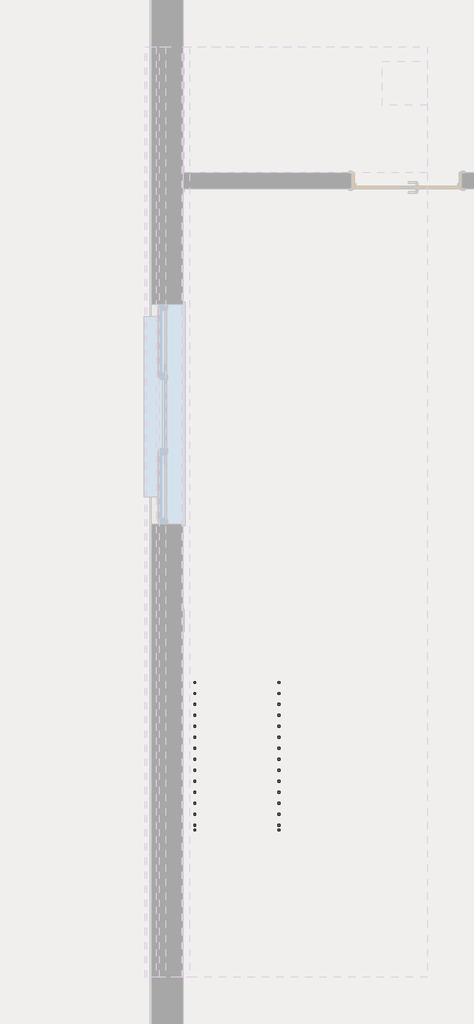
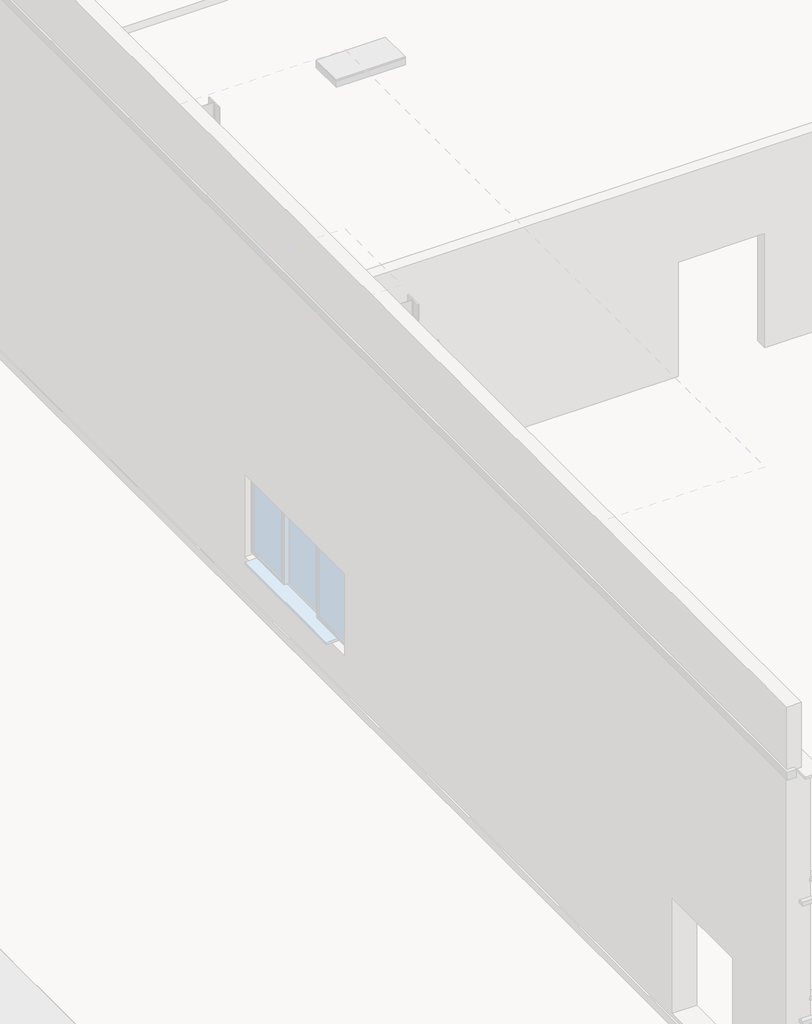
# One storey, part 7 of 13: 2 railings.
"""IFC4 building model written with IfcOpenShell, lengths in millimetres."""

from ifc_helpers import new_model, si_unit, frame, origin, place, context, project, spatial, polyline, outline, extrude, faceted_brep, element, save

model = new_model("IFC4")

# Units and contexts
model_context = context("Model", 3, world=origin())
ifc_project = project(units=[si_unit("LENGTHUNIT", "METRE", prefix="MILLI")], contexts=[model_context])

# Site, building, storey
site = spatial("IfcSite", under=ifc_project)
building = spatial("IfcBuilding", under=site)
storey = spatial("IfcBuildingStorey", under=building, Name="L0 - Ground Floor (Shadows On)", Elevation=0.0)

# Railings
placement = place(None, origin())
element("IfcRailing", 1, ObjectType="1100mm", at=placement, inside=storey, context=model_context, shape_type="SolidModel", body=[
    faceted_brep([(-5716.2916692, -13929.5546689, 1266.6666667), (-5716.2916692, -13929.5546689, 1209.4687214), (-5666.2916692, -13929.5546689, 1209.4687214), (-5666.2916692, -13929.5546689, 1266.6666667), (-5716.2916692, -11829.5546689, 2433.3333333), (-5716.2916692, -11816.5983675, 2383.3333333), (-5666.2916692, -11816.5983675, 2383.3333333), (-5666.2916692, -11829.5546689, 2433.3333333), (-5716.2916692, -10929.5546689, 2433.3333333), (-5716.2916692, -10916.5983675, 2383.3333333), (-5666.2916692, -10916.5983675, 2383.3333333), (-5666.2916692, -10929.5546689, 2433.3333333), (-5716.2916692, -8529.5546689, 3766.6666667), (-5716.2916692, -8516.5983675, 3716.6666667), (-5666.2916692, -8516.5983675, 3716.6666667), (-5666.2916692, -8529.5546689, 3766.6666667), (-5716.2916692, -7629.5546689, 3766.6666667), (-5716.2916692, -7616.5983675, 3716.6666667), (-5666.2916692, -7616.5983675, 3716.6666667), (-5666.2916692, -7629.5546689, 3766.6666667), (-5716.2916692, -5229.5546689, 5100.0), (-5666.2916692, -5229.5546689, 5100.0), (-5666.2916692, -5229.5546689, 5042.8020548), (-5716.2916692, -5229.5546689, 5042.8020548)], [[[0, 1, 2, 3]], [[1, 0, 4, 5]], [[2, 1, 5, 6]], [[3, 2, 6, 7]], [[0, 3, 7, 4]], [[5, 4, 8, 9]], [[6, 5, 9, 10]], [[7, 6, 10, 11]], [[4, 7, 11, 8]], [[9, 8, 12, 13]], [[10, 9, 13, 14]], [[11, 10, 14, 15]], [[8, 11, 15, 12]], [[13, 12, 16, 17]], [[14, 13, 17, 18]], [[15, 14, 18, 19]], [[12, 15, 19, 16]], [[20, 21, 22, 23]], [[17, 16, 20, 23]], [[18, 17, 23, 22]], [[19, 18, 22, 21]], [[16, 19, 21, 20]]]),
    extrude(outline(polyline([(-5317.0546689, 3833.3333333), (-5317.0546689, 4994.1909437), (-5292.0546689, 5008.0798326), (-5292.0546689, 3833.3333333), (-5317.0546689, 3833.3333333)])), frame((-5703.7916692, 0.0, 0.0), z_axis=(1.0, 0.0, 0.0), x_axis=(0.0, 1.0, 0.0)), (0.0, 0.0, 1.0), 25.0),
    extrude(outline(polyline([(-5467.0546689, 3833.3333333), (-5467.0546689, 4910.8576103), (-5442.0546689, 4924.7464992), (-5442.0546689, 3833.3333333), (-5467.0546689, 3833.3333333)])), frame((-5703.7916692, 0.0, 0.0), z_axis=(1.0, 0.0, 0.0), x_axis=(0.0, 1.0, 0.0)), (0.0, 0.0, 1.0), 25.0),
    extrude(outline(polyline([(-5617.0546689, 3666.6666667), (-5617.0546689, 4827.524277), (-5592.0546689, 4841.4131659), (-5592.0546689, 3666.6666667), (-5617.0546689, 3666.6666667)])), frame((-5703.7916692, 0.0, 0.0), z_axis=(1.0, 0.0, 0.0), x_axis=(0.0, 1.0, 0.0)), (0.0, 0.0, 1.0), 25.0),
    extrude(outline(polyline([(-5767.0546689, 3666.6666667), (-5767.0546689, 4744.1909437), (-5742.0546689, 4758.0798326), (-5742.0546689, 3666.6666667), (-5767.0546689, 3666.6666667)])), frame((-5703.7916692, 0.0, 0.0), z_axis=(1.0, 0.0, 0.0), x_axis=(0.0, 1.0, 0.0)), (0.0, 0.0, 1.0), 25.0),
    extrude(outline(polyline([(-5917.0546689, 3500.0), (-5917.0546689, 4660.8576103), (-5892.0546689, 4674.7464992), (-5892.0546689, 3500.0), (-5917.0546689, 3500.0)])), frame((-5703.7916692, 0.0, 0.0), z_axis=(1.0, 0.0, 0.0), x_axis=(0.0, 1.0, 0.0)), (0.0, 0.0, 1.0), 25.0),
    extrude(outline(polyline([(-6067.0546689, 3500.0), (-6067.0546689, 4577.524277), (-6042.0546689, 4591.4131659), (-6042.0546689, 3500.0), (-6067.0546689, 3500.0)])), frame((-5703.7916692, 0.0, 0.0), z_axis=(1.0, 0.0, 0.0), x_axis=(0.0, 1.0, 0.0)), (0.0, 0.0, 1.0), 25.0),
    extrude(outline(polyline([(-6217.0546689, 3333.3333333), (-6217.0546689, 4494.1909437), (-6192.0546689, 4508.0798326), (-6192.0546689, 3333.3333333), (-6217.0546689, 3333.3333333)])), frame((-5703.7916692, 0.0, 0.0), z_axis=(1.0, 0.0, 0.0), x_axis=(0.0, 1.0, 0.0)), (0.0, 0.0, 1.0), 25.0),
    extrude(outline(polyline([(-6367.0546689, 3333.3333333), (-6367.0546689, 4410.8576103), (-6342.0546689, 4424.7464992), (-6342.0546689, 3333.3333333), (-6367.0546689, 3333.3333333)])), frame((-5703.7916692, 0.0, 0.0), z_axis=(1.0, 0.0, 0.0), x_axis=(0.0, 1.0, 0.0)), (0.0, 0.0, 1.0), 25.0),
    extrude(outline(polyline([(-6517.0546689, 3166.6666667), (-6517.0546689, 4327.524277), (-6492.0546689, 4341.4131659), (-6492.0546689, 3166.6666667), (-6517.0546689, 3166.6666667)])), frame((-5703.7916692, 0.0, 0.0), z_axis=(1.0, 0.0, 0.0), x_axis=(0.0, 1.0, 0.0)), (0.0, 0.0, 1.0), 25.0),
    extrude(outline(polyline([(-6667.0546689, 3166.6666667), (-6667.0546689, 4244.1909437), (-6642.0546689, 4258.0798326), (-6642.0546689, 3166.6666667), (-6667.0546689, 3166.6666667)])), frame((-5703.7916692, 0.0, 0.0), z_axis=(1.0, 0.0, 0.0), x_axis=(0.0, 1.0, 0.0)), (0.0, 0.0, 1.0), 25.0),
    extrude(outline(polyline([(-6817.0546689, 3000.0), (-6817.0546689, 4160.8576103), (-6792.0546689, 4174.7464992), (-6792.0546689, 3000.0), (-6817.0546689, 3000.0)])), frame((-5703.7916692, 0.0, 0.0), z_axis=(1.0, 0.0, 0.0), x_axis=(0.0, 1.0, 0.0)), (0.0, 0.0, 1.0), 25.0),
    extrude(outline(polyline([(-6967.0546689, 3000.0), (-6967.0546689, 4077.524277), (-6942.0546689, 4091.4131659), (-6942.0546689, 3000.0), (-6967.0546689, 3000.0)])), frame((-5703.7916692, 0.0, 0.0), z_axis=(1.0, 0.0, 0.0), x_axis=(0.0, 1.0, 0.0)), (0.0, 0.0, 1.0), 25.0),
    extrude(outline(polyline([(-7117.0546689, 2833.3333333), (-7117.0546689, 3994.1909437), (-7092.0546689, 4008.0798326), (-7092.0546689, 2833.3333333), (-7117.0546689, 2833.3333333)])), frame((-5703.7916692, 0.0, 0.0), z_axis=(1.0, 0.0, 0.0), x_axis=(0.0, 1.0, 0.0)), (0.0, 0.0, 1.0), 25.0),
    extrude(outline(polyline([(-7267.0546689, 2833.3333333), (-7267.0546689, 3910.8576103), (-7242.0546689, 3924.7464992), (-7242.0546689, 2833.3333333), (-7267.0546689, 2833.3333333)])), frame((-5703.7916692, 0.0, 0.0), z_axis=(1.0, 0.0, 0.0), x_axis=(0.0, 1.0, 0.0)), (0.0, 0.0, 1.0), 25.0),
    extrude(outline(polyline([(-7417.0546689, 2666.6666667), (-7417.0546689, 3827.524277), (-7392.0546689, 3841.4131659), (-7392.0546689, 2666.6666667), (-7417.0546689, 2666.6666667)])), frame((-5703.7916692, 0.0, 0.0), z_axis=(1.0, 0.0, 0.0), x_axis=(0.0, 1.0, 0.0)), (0.0, 0.0, 1.0), 25.0),
    extrude(outline(polyline([(-7567.0546689, 2666.6666667), (-7567.0546689, 3744.1909437), (-7542.0546689, 3758.0798326), (-7542.0546689, 2666.6666667), (-7567.0546689, 2666.6666667)])), frame((-5703.7916692, 0.0, 0.0), z_axis=(1.0, 0.0, 0.0), x_axis=(0.0, 1.0, 0.0)), (0.0, 0.0, 1.0), 25.0),
    extrude(outline(polyline([(-5678.7916692, -7717.0546689), (-5703.7916692, -7717.0546689), (-5703.7916692, -7692.0546689), (-5678.7916692, -7692.0546689), (-5678.7916692, -7717.0546689)])), frame((0.0, 0.0, 2666.6666667), z_axis=(0.0, 0.0, 1.0), x_axis=(1.0, 0.0, 0.0)), (0.0, 0.0, 1.0), 1050.0),
    extrude(outline(polyline([(-5678.7916692, -7867.0546689), (-5703.7916692, -7867.0546689), (-5703.7916692, -7842.0546689), (-5678.7916692, -7842.0546689), (-5678.7916692, -7867.0546689)])), frame((0.0, 0.0, 2666.6666667), z_axis=(0.0, 0.0, 1.0), x_axis=(1.0, 0.0, 0.0)), (0.0, 0.0, 1.0), 1050.0),
    extrude(outline(polyline([(-5678.7916692, -8017.0546689), (-5703.7916692, -8017.0546689), (-5703.7916692, -7992.0546689), (-5678.7916692, -7992.0546689), (-5678.7916692, -8017.0546689)])), frame((0.0, 0.0, 2666.6666667), z_axis=(0.0, 0.0, 1.0), x_axis=(1.0, 0.0, 0.0)), (0.0, 0.0, 1.0), 1050.0),
    extrude(outline(polyline([(-5678.7916692, -8167.0546689), (-5703.7916692, -8167.0546689), (-5703.7916692, -8142.0546689), (-5678.7916692, -8142.0546689), (-5678.7916692, -8167.0546689)])), frame((0.0, 0.0, 2666.6666667), z_axis=(0.0, 0.0, 1.0), x_axis=(1.0, 0.0, 0.0)), (0.0, 0.0, 1.0), 1050.0),
    extrude(outline(polyline([(-5678.7916692, -8317.0546689), (-5703.7916692, -8317.0546689), (-5703.7916692, -8292.0546689), (-5678.7916692, -8292.0546689), (-5678.7916692, -8317.0546689)])), frame((0.0, 0.0, 2666.6666667), z_axis=(0.0, 0.0, 1.0), x_axis=(1.0, 0.0, 0.0)), (0.0, 0.0, 1.0), 1050.0),
    extrude(outline(polyline([(-5678.7916692, -8467.0546689), (-5703.7916692, -8467.0546689), (-5703.7916692, -8442.0546689), (-5678.7916692, -8442.0546689), (-5678.7916692, -8467.0546689)])), frame((0.0, 0.0, 2666.6666667), z_axis=(0.0, 0.0, 1.0), x_axis=(1.0, 0.0, 0.0)), (0.0, 0.0, 1.0), 1050.0),
    extrude(outline(polyline([(-8617.0546689, 2500.0), (-8617.0546689, 3660.8576103), (-8592.0546689, 3674.7464992), (-8592.0546689, 2500.0), (-8617.0546689, 2500.0)])), frame((-5703.7916692, 0.0, 0.0), z_axis=(1.0, 0.0, 0.0), x_axis=(0.0, 1.0, 0.0)), (0.0, 0.0, 1.0), 25.0),
    extrude(outline(polyline([(-8767.0546689, 2500.0), (-8767.0546689, 3577.524277), (-8742.0546689, 3591.4131659), (-8742.0546689, 2500.0), (-8767.0546689, 2500.0)])), frame((-5703.7916692, 0.0, 0.0), z_axis=(1.0, 0.0, 0.0), x_axis=(0.0, 1.0, 0.0)), (0.0, 0.0, 1.0), 25.0),
    extrude(outline(polyline([(-8917.0546689, 2333.3333333), (-8917.0546689, 3494.1909437), (-8892.0546689, 3508.0798326), (-8892.0546689, 2333.3333333), (-8917.0546689, 2333.3333333)])), frame((-5703.7916692, 0.0, 0.0), z_axis=(1.0, 0.0, 0.0), x_axis=(0.0, 1.0, 0.0)), (0.0, 0.0, 1.0), 25.0),
    extrude(outline(polyline([(-9067.0546689, 2333.3333333), (-9067.0546689, 3410.8576103), (-9042.0546689, 3424.7464992), (-9042.0546689, 2333.3333333), (-9067.0546689, 2333.3333333)])), frame((-5703.7916692, 0.0, 0.0), z_axis=(1.0, 0.0, 0.0), x_axis=(0.0, 1.0, 0.0)), (0.0, 0.0, 1.0), 25.0),
    extrude(outline(polyline([(-9217.0546689, 2166.6666667), (-9217.0546689, 3327.524277), (-9192.0546689, 3341.4131659), (-9192.0546689, 2166.6666667), (-9217.0546689, 2166.6666667)])), frame((-5703.7916692, 0.0, 0.0), z_axis=(1.0, 0.0, 0.0), x_axis=(0.0, 1.0, 0.0)), (0.0, 0.0, 1.0), 25.0),
    extrude(outline(polyline([(-9367.0546689, 2166.6666667), (-9367.0546689, 3244.1909437), (-9342.0546689, 3258.0798326), (-9342.0546689, 2166.6666667), (-9367.0546689, 2166.6666667)])), frame((-5703.7916692, 0.0, 0.0), z_axis=(1.0, 0.0, 0.0), x_axis=(0.0, 1.0, 0.0)), (0.0, 0.0, 1.0), 25.0),
    extrude(outline(polyline([(-9517.0546689, 2000.0), (-9517.0546689, 3160.8576103), (-9492.0546689, 3174.7464992), (-9492.0546689, 2000.0), (-9517.0546689, 2000.0)])), frame((-5703.7916692, 0.0, 0.0), z_axis=(1.0, 0.0, 0.0), x_axis=(0.0, 1.0, 0.0)), (0.0, 0.0, 1.0), 25.0),
    extrude(outline(polyline([(-9667.0546689, 2000.0), (-9667.0546689, 3077.524277), (-9642.0546689, 3091.4131659), (-9642.0546689, 2000.0), (-9667.0546689, 2000.0)])), frame((-5703.7916692, 0.0, 0.0), z_axis=(1.0, 0.0, 0.0), x_axis=(0.0, 1.0, 0.0)), (0.0, 0.0, 1.0), 25.0),
    extrude(outline(polyline([(-9817.0546689, 1833.3333333), (-9817.0546689, 2994.1909437), (-9792.0546689, 3008.0798326), (-9792.0546689, 1833.3333333), (-9817.0546689, 1833.3333333)])), frame((-5703.7916692, 0.0, 0.0), z_axis=(1.0, 0.0, 0.0), x_axis=(0.0, 1.0, 0.0)), (0.0, 0.0, 1.0), 25.0),
    extrude(outline(polyline([(-9967.0546689, 1833.3333333), (-9967.0546689, 2910.8576103), (-9942.0546689, 2924.7464992), (-9942.0546689, 1833.3333333), (-9967.0546689, 1833.3333333)])), frame((-5703.7916692, 0.0, 0.0), z_axis=(1.0, 0.0, 0.0), x_axis=(0.0, 1.0, 0.0)), (0.0, 0.0, 1.0), 25.0),
    extrude(outline(polyline([(-10117.0546689, 1666.6666667), (-10117.0546689, 2827.524277), (-10092.0546689, 2841.4131659), (-10092.0546689, 1666.6666667), (-10117.0546689, 1666.6666667)])), frame((-5703.7916692, 0.0, 0.0), z_axis=(1.0, 0.0, 0.0), x_axis=(0.0, 1.0, 0.0)), (0.0, 0.0, 1.0), 25.0),
    extrude(outline(polyline([(-10267.0546689, 1666.6666667), (-10267.0546689, 2744.1909437), (-10242.0546689, 2758.0798326), (-10242.0546689, 1666.6666667), (-10267.0546689, 1666.6666667)])), frame((-5703.7916692, 0.0, 0.0), z_axis=(1.0, 0.0, 0.0), x_axis=(0.0, 1.0, 0.0)), (0.0, 0.0, 1.0), 25.0),
    extrude(outline(polyline([(-10417.0546689, 1500.0), (-10417.0546689, 2660.8576103), (-10392.0546689, 2674.7464992), (-10392.0546689, 1500.0), (-10417.0546689, 1500.0)])), frame((-5703.7916692, 0.0, 0.0), z_axis=(1.0, 0.0, 0.0), x_axis=(0.0, 1.0, 0.0)), (0.0, 0.0, 1.0), 25.0),
    extrude(outline(polyline([(-10567.0546689, 1500.0), (-10567.0546689, 2577.524277), (-10542.0546689, 2591.4131659), (-10542.0546689, 1500.0), (-10567.0546689, 1500.0)])), frame((-5703.7916692, 0.0, 0.0), z_axis=(1.0, 0.0, 0.0), x_axis=(0.0, 1.0, 0.0)), (0.0, 0.0, 1.0), 25.0),
    extrude(outline(polyline([(-10717.0546689, 1333.3333333), (-10717.0546689, 2494.1909437), (-10692.0546689, 2508.0798326), (-10692.0546689, 1333.3333333), (-10717.0546689, 1333.3333333)])), frame((-5703.7916692, 0.0, 0.0), z_axis=(1.0, 0.0, 0.0), x_axis=(0.0, 1.0, 0.0)), (0.0, 0.0, 1.0), 25.0),
    extrude(outline(polyline([(-10867.0546689, 1333.3333333), (-10867.0546689, 2410.8576103), (-10842.0546689, 2424.7464992), (-10842.0546689, 1333.3333333), (-10867.0546689, 1333.3333333)])), frame((-5703.7916692, 0.0, 0.0), z_axis=(1.0, 0.0, 0.0), x_axis=(0.0, 1.0, 0.0)), (0.0, 0.0, 1.0), 25.0),
    extrude(outline(polyline([(-5678.7916692, -11017.0546689), (-5703.7916692, -11017.0546689), (-5703.7916692, -10992.0546689), (-5678.7916692, -10992.0546689), (-5678.7916692, -11017.0546689)])), frame((0.0, 0.0, 1333.3333333), z_axis=(0.0, 0.0, 1.0), x_axis=(1.0, 0.0, 0.0)), (0.0, 0.0, 1.0), 1050.0),
    extrude(outline(polyline([(-5678.7916692, -11167.0546689), (-5703.7916692, -11167.0546689), (-5703.7916692, -11142.0546689), (-5678.7916692, -11142.0546689), (-5678.7916692, -11167.0546689)])), frame((0.0, 0.0, 1333.3333333), z_axis=(0.0, 0.0, 1.0), x_axis=(1.0, 0.0, 0.0)), (0.0, 0.0, 1.0), 1050.0),
    extrude(outline(polyline([(-5678.7916692, -11317.0546689), (-5703.7916692, -11317.0546689), (-5703.7916692, -11292.0546689), (-5678.7916692, -11292.0546689), (-5678.7916692, -11317.0546689)])), frame((0.0, 0.0, 1333.3333333), z_axis=(0.0, 0.0, 1.0), x_axis=(1.0, 0.0, 0.0)), (0.0, 0.0, 1.0), 1050.0),
    extrude(outline(polyline([(-5678.7916692, -11467.0546689), (-5703.7916692, -11467.0546689), (-5703.7916692, -11442.0546689), (-5678.7916692, -11442.0546689), (-5678.7916692, -11467.0546689)])), frame((0.0, 0.0, 1333.3333333), z_axis=(0.0, 0.0, 1.0), x_axis=(1.0, 0.0, 0.0)), (0.0, 0.0, 1.0), 1050.0),
    extrude(outline(polyline([(-5678.7916692, -11617.0546689), (-5703.7916692, -11617.0546689), (-5703.7916692, -11592.0546689), (-5678.7916692, -11592.0546689), (-5678.7916692, -11617.0546689)])), frame((0.0, 0.0, 1333.3333333), z_axis=(0.0, 0.0, 1.0), x_axis=(1.0, 0.0, 0.0)), (0.0, 0.0, 1.0), 1050.0),
    extrude(outline(polyline([(-5678.7916692, -11767.0546689), (-5703.7916692, -11767.0546689), (-5703.7916692, -11742.0546689), (-5678.7916692, -11742.0546689), (-5678.7916692, -11767.0546689)])), frame((0.0, 0.0, 1333.3333333), z_axis=(0.0, 0.0, 1.0), x_axis=(1.0, 0.0, 0.0)), (0.0, 0.0, 1.0), 1050.0),
    extrude(outline(polyline([(-11917.0546689, 1166.6666667), (-11917.0546689, 2327.524277), (-11892.0546689, 2341.4131659), (-11892.0546689, 1166.6666667), (-11917.0546689, 1166.6666667)])), frame((-5703.7916692, 0.0, 0.0), z_axis=(1.0, 0.0, 0.0), x_axis=(0.0, 1.0, 0.0)), (0.0, 0.0, 1.0), 25.0),
    extrude(outline(polyline([(-12067.0546689, 1166.6666667), (-12067.0546689, 2244.1909437), (-12042.0546689, 2258.0798326), (-12042.0546689, 1166.6666667), (-12067.0546689, 1166.6666667)])), frame((-5703.7916692, 0.0, 0.0), z_axis=(1.0, 0.0, 0.0), x_axis=(0.0, 1.0, 0.0)), (0.0, 0.0, 1.0), 25.0),
    extrude(outline(polyline([(-12217.0546689, 1000.0), (-12217.0546689, 2160.8576103), (-12192.0546689, 2174.7464992), (-12192.0546689, 1000.0), (-12217.0546689, 1000.0)])), frame((-5703.7916692, 0.0, 0.0), z_axis=(1.0, 0.0, 0.0), x_axis=(0.0, 1.0, 0.0)), (0.0, 0.0, 1.0), 25.0),
    extrude(outline(polyline([(-12367.0546689, 1000.0), (-12367.0546689, 2077.524277), (-12342.0546689, 2091.4131659), (-12342.0546689, 1000.0), (-12367.0546689, 1000.0)])), frame((-5703.7916692, 0.0, 0.0), z_axis=(1.0, 0.0, 0.0), x_axis=(0.0, 1.0, 0.0)), (0.0, 0.0, 1.0), 25.0),
    extrude(outline(polyline([(-12517.0546689, 833.3333333), (-12517.0546689, 1994.1909437), (-12492.0546689, 2008.0798326), (-12492.0546689, 833.3333333), (-12517.0546689, 833.3333333)])), frame((-5703.7916692, 0.0, 0.0), z_axis=(1.0, 0.0, 0.0), x_axis=(0.0, 1.0, 0.0)), (0.0, 0.0, 1.0), 25.0),
    extrude(outline(polyline([(-12667.0546689, 833.3333333), (-12667.0546689, 1910.8576103), (-12642.0546689, 1924.7464992), (-12642.0546689, 833.3333333), (-12667.0546689, 833.3333333)])), frame((-5703.7916692, 0.0, 0.0), z_axis=(1.0, 0.0, 0.0), x_axis=(0.0, 1.0, 0.0)), (0.0, 0.0, 1.0), 25.0),
    extrude(outline(polyline([(-12817.0546689, 666.6666667), (-12817.0546689, 1827.524277), (-12792.0546689, 1841.4131659), (-12792.0546689, 666.6666667), (-12817.0546689, 666.6666667)])), frame((-5703.7916692, 0.0, 0.0), z_axis=(1.0, 0.0, 0.0), x_axis=(0.0, 1.0, 0.0)), (0.0, 0.0, 1.0), 25.0),
    extrude(outline(polyline([(-12967.0546689, 666.6666667), (-12967.0546689, 1744.1909437), (-12942.0546689, 1758.0798326), (-12942.0546689, 666.6666667), (-12967.0546689, 666.6666667)])), frame((-5703.7916692, 0.0, 0.0), z_axis=(1.0, 0.0, 0.0), x_axis=(0.0, 1.0, 0.0)), (0.0, 0.0, 1.0), 25.0),
    extrude(outline(polyline([(-13117.0546689, 500.0), (-13117.0546689, 1660.8576103), (-13092.0546689, 1674.7464992), (-13092.0546689, 500.0), (-13117.0546689, 500.0)])), frame((-5703.7916692, 0.0, 0.0), z_axis=(1.0, 0.0, 0.0), x_axis=(0.0, 1.0, 0.0)), (0.0, 0.0, 1.0), 25.0),
    extrude(outline(polyline([(-13267.0546689, 500.0), (-13267.0546689, 1577.524277), (-13242.0546689, 1591.4131659), (-13242.0546689, 500.0), (-13267.0546689, 500.0)])), frame((-5703.7916692, 0.0, 0.0), z_axis=(1.0, 0.0, 0.0), x_axis=(0.0, 1.0, 0.0)), (0.0, 0.0, 1.0), 25.0),
    extrude(outline(polyline([(-13417.0546689, 333.3333333), (-13417.0546689, 1494.1909437), (-13392.0546689, 1508.0798326), (-13392.0546689, 333.3333333), (-13417.0546689, 333.3333333)])), frame((-5703.7916692, 0.0, 0.0), z_axis=(1.0, 0.0, 0.0), x_axis=(0.0, 1.0, 0.0)), (0.0, 0.0, 1.0), 25.0),
    extrude(outline(polyline([(-13567.0546689, 333.3333333), (-13567.0546689, 1410.8576103), (-13542.0546689, 1424.7464992), (-13542.0546689, 333.3333333), (-13567.0546689, 333.3333333)])), frame((-5703.7916692, 0.0, 0.0), z_axis=(1.0, 0.0, 0.0), x_axis=(0.0, 1.0, 0.0)), (0.0, 0.0, 1.0), 25.0),
    extrude(outline(polyline([(-13717.0546689, 166.6666667), (-13717.0546689, 1327.524277), (-13692.0546689, 1341.4131659), (-13692.0546689, 166.6666667), (-13717.0546689, 166.6666667)])), frame((-5703.7916692, 0.0, 0.0), z_axis=(1.0, 0.0, 0.0), x_axis=(0.0, 1.0, 0.0)), (0.0, 0.0, 1.0), 25.0),
    extrude(outline(polyline([(-13867.0546689, 166.6666667), (-13867.0546689, 1244.1909437), (-13842.0546689, 1258.0798326), (-13842.0546689, 166.6666667), (-13867.0546689, 166.6666667)])), frame((-5703.7916692, 0.0, 0.0), z_axis=(1.0, 0.0, 0.0), x_axis=(0.0, 1.0, 0.0)), (0.0, 0.0, 1.0), 25.0),
    extrude(outline(polyline([(-5678.7916692, -7642.0546689), (-5703.7916692, -7642.0546689), (-5703.7916692, -7617.0546689), (-5678.7916692, -7617.0546689), (-5678.7916692, -7642.0546689)])), frame((0.0, 0.0, 2666.6666667), z_axis=(0.0, 0.0, 1.0), x_axis=(1.0, 0.0, 0.0)), (0.0, 0.0, 1.0), 1050.0),
    extrude(outline(polyline([(-8542.0546689, 2666.6666667), (-8542.0546689, 3702.524277), (-8517.0546689, 3716.4131659), (-8517.0546689, 2666.6666667), (-8542.0546689, 2666.6666667)])), frame((-5703.7916692, 0.0, 0.0), z_axis=(1.0, 0.0, 0.0), x_axis=(0.0, 1.0, 0.0)), (0.0, 0.0, 1.0), 25.0),
    extrude(outline(polyline([(-5678.7916692, -10942.0546689), (-5703.7916692, -10942.0546689), (-5703.7916692, -10917.0546689), (-5678.7916692, -10917.0546689), (-5678.7916692, -10942.0546689)])), frame((0.0, 0.0, 1333.3333333), z_axis=(0.0, 0.0, 1.0), x_axis=(1.0, 0.0, 0.0)), (0.0, 0.0, 1.0), 1050.0),
    extrude(outline(polyline([(-11842.0546689, 1333.3333333), (-11842.0546689, 2369.1909437), (-11817.0546689, 2383.0798326), (-11817.0546689, 1333.3333333), (-11842.0546689, 1333.3333333)])), frame((-5703.7916692, 0.0, 0.0), z_axis=(1.0, 0.0, 0.0), x_axis=(0.0, 1.0, 0.0)), (0.0, 0.0, 1.0), 25.0),
    extrude(outline(polyline([(-5254.5546689, 3833.3333333), (-5254.5546689, 5028.9131659), (-5229.5546689, 5042.8020548), (-5229.5546689, 3833.3333333), (-5254.5546689, 3833.3333333)])), frame((-5703.7916692, 0.0, 0.0), z_axis=(1.0, 0.0, 0.0), x_axis=(0.0, 1.0, 0.0)), (0.0, 0.0, 1.0), 25.0),
    extrude(outline(polyline([(-13929.5546689, 166.6666667), (-13929.5546689, 1209.4687214), (-13904.5546689, 1223.3576103), (-13904.5546689, 166.6666667), (-13929.5546689, 166.6666667)])), frame((-5703.7916692, 0.0, 0.0), z_axis=(1.0, 0.0, 0.0), x_axis=(0.0, 1.0, 0.0)), (0.0, 0.0, 1.0), 25.0),
])
element("IfcRailing", 2, ObjectType="1100mm", at=placement, inside=storey, context=model_context, shape_type="SolidModel", body=[
    faceted_brep([(-6865.4916692, -13929.5546689, 1266.6666667), (-6865.4916692, -13929.5546689, 1209.4687214), (-6815.4916692, -13929.5546689, 1209.4687214), (-6815.4916692, -13929.5546689, 1266.6666667), (-6865.4916692, -11829.5546689, 2433.3333333), (-6865.4916692, -11816.5983675, 2383.3333333), (-6815.4916692, -11816.5983675, 2383.3333333), (-6815.4916692, -11829.5546689, 2433.3333333), (-6865.4916692, -10929.5546689, 2433.3333333), (-6865.4916692, -10916.5983675, 2383.3333333), (-6815.4916692, -10916.5983675, 2383.3333333), (-6815.4916692, -10929.5546689, 2433.3333333), (-6865.4916692, -8529.5546689, 3766.6666667), (-6865.4916692, -8516.5983675, 3716.6666667), (-6815.4916692, -8516.5983675, 3716.6666667), (-6815.4916692, -8529.5546689, 3766.6666667), (-6865.4916692, -7629.5546689, 3766.6666667), (-6865.4916692, -7616.5983675, 3716.6666667), (-6815.4916692, -7616.5983675, 3716.6666667), (-6815.4916692, -7629.5546689, 3766.6666667), (-6865.4916692, -5229.5546689, 5100.0), (-6815.4916692, -5229.5546689, 5100.0), (-6815.4916692, -5229.5546689, 5042.8020548), (-6865.4916692, -5229.5546689, 5042.8020548)], [[[0, 1, 2, 3]], [[1, 0, 4, 5]], [[2, 1, 5, 6]], [[3, 2, 6, 7]], [[0, 3, 7, 4]], [[5, 4, 8, 9]], [[6, 5, 9, 10]], [[7, 6, 10, 11]], [[4, 7, 11, 8]], [[9, 8, 12, 13]], [[10, 9, 13, 14]], [[11, 10, 14, 15]], [[8, 11, 15, 12]], [[13, 12, 16, 17]], [[14, 13, 17, 18]], [[15, 14, 18, 19]], [[12, 15, 19, 16]], [[20, 21, 22, 23]], [[17, 16, 20, 23]], [[18, 17, 23, 22]], [[19, 18, 22, 21]], [[16, 19, 21, 20]]]),
    extrude(outline(polyline([(-5317.0546689, 4994.1909437), (-5292.0546689, 5008.0798326), (-5292.0546689, 3833.3333333), (-5317.0546689, 3833.3333333), (-5317.0546689, 4994.1909437)])), frame((-6852.9916692, 0.0, 0.0), z_axis=(1.0, 0.0, 0.0), x_axis=(0.0, 1.0, 0.0)), (0.0, 0.0, 1.0), 25.0),
    extrude(outline(polyline([(-5467.0546689, 4910.8576103), (-5442.0546689, 4924.7464992), (-5442.0546689, 3833.3333333), (-5467.0546689, 3833.3333333), (-5467.0546689, 4910.8576103)])), frame((-6852.9916692, 0.0, 0.0), z_axis=(1.0, 0.0, 0.0), x_axis=(0.0, 1.0, 0.0)), (0.0, 0.0, 1.0), 25.0),
    extrude(outline(polyline([(-5617.0546689, 4827.524277), (-5592.0546689, 4841.4131659), (-5592.0546689, 3666.6666667), (-5617.0546689, 3666.6666667), (-5617.0546689, 4827.524277)])), frame((-6852.9916692, 0.0, 0.0), z_axis=(1.0, 0.0, 0.0), x_axis=(0.0, 1.0, 0.0)), (0.0, 0.0, 1.0), 25.0),
    extrude(outline(polyline([(-5767.0546689, 4744.1909437), (-5742.0546689, 4758.0798326), (-5742.0546689, 3666.6666667), (-5767.0546689, 3666.6666667), (-5767.0546689, 4744.1909437)])), frame((-6852.9916692, 0.0, 0.0), z_axis=(1.0, 0.0, 0.0), x_axis=(0.0, 1.0, 0.0)), (0.0, 0.0, 1.0), 25.0),
    extrude(outline(polyline([(-5917.0546689, 4660.8576103), (-5892.0546689, 4674.7464992), (-5892.0546689, 3500.0), (-5917.0546689, 3500.0), (-5917.0546689, 4660.8576103)])), frame((-6852.9916692, 0.0, 0.0), z_axis=(1.0, 0.0, 0.0), x_axis=(0.0, 1.0, 0.0)), (0.0, 0.0, 1.0), 25.0),
    extrude(outline(polyline([(-6067.0546689, 4577.524277), (-6042.0546689, 4591.4131659), (-6042.0546689, 3500.0), (-6067.0546689, 3500.0), (-6067.0546689, 4577.524277)])), frame((-6852.9916692, 0.0, 0.0), z_axis=(1.0, 0.0, 0.0), x_axis=(0.0, 1.0, 0.0)), (0.0, 0.0, 1.0), 25.0),
    extrude(outline(polyline([(-6217.0546689, 4494.1909437), (-6192.0546689, 4508.0798326), (-6192.0546689, 3333.3333333), (-6217.0546689, 3333.3333333), (-6217.0546689, 4494.1909437)])), frame((-6852.9916692, 0.0, 0.0), z_axis=(1.0, 0.0, 0.0), x_axis=(0.0, 1.0, 0.0)), (0.0, 0.0, 1.0), 25.0),
    extrude(outline(polyline([(-6367.0546689, 4410.8576103), (-6342.0546689, 4424.7464992), (-6342.0546689, 3333.3333333), (-6367.0546689, 3333.3333333), (-6367.0546689, 4410.8576103)])), frame((-6852.9916692, 0.0, 0.0), z_axis=(1.0, 0.0, 0.0), x_axis=(0.0, 1.0, 0.0)), (0.0, 0.0, 1.0), 25.0),
    extrude(outline(polyline([(-6517.0546689, 4327.524277), (-6492.0546689, 4341.4131659), (-6492.0546689, 3166.6666667), (-6517.0546689, 3166.6666667), (-6517.0546689, 4327.524277)])), frame((-6852.9916692, 0.0, 0.0), z_axis=(1.0, 0.0, 0.0), x_axis=(0.0, 1.0, 0.0)), (0.0, 0.0, 1.0), 25.0),
    extrude(outline(polyline([(-6667.0546689, 4244.1909437), (-6642.0546689, 4258.0798326), (-6642.0546689, 3166.6666667), (-6667.0546689, 3166.6666667), (-6667.0546689, 4244.1909437)])), frame((-6852.9916692, 0.0, 0.0), z_axis=(1.0, 0.0, 0.0), x_axis=(0.0, 1.0, 0.0)), (0.0, 0.0, 1.0), 25.0),
    extrude(outline(polyline([(-6817.0546689, 4160.8576103), (-6792.0546689, 4174.7464992), (-6792.0546689, 3000.0), (-6817.0546689, 3000.0), (-6817.0546689, 4160.8576103)])), frame((-6852.9916692, 0.0, 0.0), z_axis=(1.0, 0.0, 0.0), x_axis=(0.0, 1.0, 0.0)), (0.0, 0.0, 1.0), 25.0),
    extrude(outline(polyline([(-6967.0546689, 4077.524277), (-6942.0546689, 4091.4131659), (-6942.0546689, 3000.0), (-6967.0546689, 3000.0), (-6967.0546689, 4077.524277)])), frame((-6852.9916692, 0.0, 0.0), z_axis=(1.0, 0.0, 0.0), x_axis=(0.0, 1.0, 0.0)), (0.0, 0.0, 1.0), 25.0),
    extrude(outline(polyline([(-7117.0546689, 3994.1909437), (-7092.0546689, 4008.0798326), (-7092.0546689, 2833.3333333), (-7117.0546689, 2833.3333333), (-7117.0546689, 3994.1909437)])), frame((-6852.9916692, 0.0, 0.0), z_axis=(1.0, 0.0, 0.0), x_axis=(0.0, 1.0, 0.0)), (0.0, 0.0, 1.0), 25.0),
    extrude(outline(polyline([(-7267.0546689, 3910.8576103), (-7242.0546689, 3924.7464992), (-7242.0546689, 2833.3333333), (-7267.0546689, 2833.3333333), (-7267.0546689, 3910.8576103)])), frame((-6852.9916692, 0.0, 0.0), z_axis=(1.0, 0.0, 0.0), x_axis=(0.0, 1.0, 0.0)), (0.0, 0.0, 1.0), 25.0),
    extrude(outline(polyline([(-7417.0546689, 3827.524277), (-7392.0546689, 3841.4131659), (-7392.0546689, 2666.6666667), (-7417.0546689, 2666.6666667), (-7417.0546689, 3827.524277)])), frame((-6852.9916692, 0.0, 0.0), z_axis=(1.0, 0.0, 0.0), x_axis=(0.0, 1.0, 0.0)), (0.0, 0.0, 1.0), 25.0),
    extrude(outline(polyline([(-7567.0546689, 3744.1909437), (-7542.0546689, 3758.0798326), (-7542.0546689, 2666.6666667), (-7567.0546689, 2666.6666667), (-7567.0546689, 3744.1909437)])), frame((-6852.9916692, 0.0, 0.0), z_axis=(1.0, 0.0, 0.0), x_axis=(0.0, 1.0, 0.0)), (0.0, 0.0, 1.0), 25.0),
    extrude(outline(polyline([(-6852.9916692, -7717.0546689), (-6852.9916692, -7692.0546689), (-6827.9916692, -7692.0546689), (-6827.9916692, -7717.0546689), (-6852.9916692, -7717.0546689)])), frame((0.0, 0.0, 2666.6666667), z_axis=(0.0, 0.0, 1.0), x_axis=(1.0, 0.0, 0.0)), (0.0, 0.0, 1.0), 1050.0),
    extrude(outline(polyline([(-6852.9916692, -7867.0546689), (-6852.9916692, -7842.0546689), (-6827.9916692, -7842.0546689), (-6827.9916692, -7867.0546689), (-6852.9916692, -7867.0546689)])), frame((0.0, 0.0, 2666.6666667), z_axis=(0.0, 0.0, 1.0), x_axis=(1.0, 0.0, 0.0)), (0.0, 0.0, 1.0), 1050.0),
    extrude(outline(polyline([(-6852.9916692, -8017.0546689), (-6852.9916692, -7992.0546689), (-6827.9916692, -7992.0546689), (-6827.9916692, -8017.0546689), (-6852.9916692, -8017.0546689)])), frame((0.0, 0.0, 2666.6666667), z_axis=(0.0, 0.0, 1.0), x_axis=(1.0, 0.0, 0.0)), (0.0, 0.0, 1.0), 1050.0),
    extrude(outline(polyline([(-6852.9916692, -8167.0546689), (-6852.9916692, -8142.0546689), (-6827.9916692, -8142.0546689), (-6827.9916692, -8167.0546689), (-6852.9916692, -8167.0546689)])), frame((0.0, 0.0, 2666.6666667), z_axis=(0.0, 0.0, 1.0), x_axis=(1.0, 0.0, 0.0)), (0.0, 0.0, 1.0), 1050.0),
    extrude(outline(polyline([(-6852.9916692, -8317.0546689), (-6852.9916692, -8292.0546689), (-6827.9916692, -8292.0546689), (-6827.9916692, -8317.0546689), (-6852.9916692, -8317.0546689)])), frame((0.0, 0.0, 2666.6666667), z_axis=(0.0, 0.0, 1.0), x_axis=(1.0, 0.0, 0.0)), (0.0, 0.0, 1.0), 1050.0),
    extrude(outline(polyline([(-6852.9916692, -8467.0546689), (-6852.9916692, -8442.0546689), (-6827.9916692, -8442.0546689), (-6827.9916692, -8467.0546689), (-6852.9916692, -8467.0546689)])), frame((0.0, 0.0, 2666.6666667), z_axis=(0.0, 0.0, 1.0), x_axis=(1.0, 0.0, 0.0)), (0.0, 0.0, 1.0), 1050.0),
    extrude(outline(polyline([(-8617.0546689, 3660.8576103), (-8592.0546689, 3674.7464992), (-8592.0546689, 2500.0), (-8617.0546689, 2500.0), (-8617.0546689, 3660.8576103)])), frame((-6852.9916692, 0.0, 0.0), z_axis=(1.0, 0.0, 0.0), x_axis=(0.0, 1.0, 0.0)), (0.0, 0.0, 1.0), 25.0),
    extrude(outline(polyline([(-8767.0546689, 3577.524277), (-8742.0546689, 3591.4131659), (-8742.0546689, 2500.0), (-8767.0546689, 2500.0), (-8767.0546689, 3577.524277)])), frame((-6852.9916692, 0.0, 0.0), z_axis=(1.0, 0.0, 0.0), x_axis=(0.0, 1.0, 0.0)), (0.0, 0.0, 1.0), 25.0),
    extrude(outline(polyline([(-8917.0546689, 3494.1909437), (-8892.0546689, 3508.0798326), (-8892.0546689, 2333.3333333), (-8917.0546689, 2333.3333333), (-8917.0546689, 3494.1909437)])), frame((-6852.9916692, 0.0, 0.0), z_axis=(1.0, 0.0, 0.0), x_axis=(0.0, 1.0, 0.0)), (0.0, 0.0, 1.0), 25.0),
    extrude(outline(polyline([(-9067.0546689, 3410.8576103), (-9042.0546689, 3424.7464992), (-9042.0546689, 2333.3333333), (-9067.0546689, 2333.3333333), (-9067.0546689, 3410.8576103)])), frame((-6852.9916692, 0.0, 0.0), z_axis=(1.0, 0.0, 0.0), x_axis=(0.0, 1.0, 0.0)), (0.0, 0.0, 1.0), 25.0),
    extrude(outline(polyline([(-9217.0546689, 3327.524277), (-9192.0546689, 3341.4131659), (-9192.0546689, 2166.6666667), (-9217.0546689, 2166.6666667), (-9217.0546689, 3327.524277)])), frame((-6852.9916692, 0.0, 0.0), z_axis=(1.0, 0.0, 0.0), x_axis=(0.0, 1.0, 0.0)), (0.0, 0.0, 1.0), 25.0),
    extrude(outline(polyline([(-9367.0546689, 3244.1909437), (-9342.0546689, 3258.0798326), (-9342.0546689, 2166.6666667), (-9367.0546689, 2166.6666667), (-9367.0546689, 3244.1909437)])), frame((-6852.9916692, 0.0, 0.0), z_axis=(1.0, 0.0, 0.0), x_axis=(0.0, 1.0, 0.0)), (0.0, 0.0, 1.0), 25.0),
    extrude(outline(polyline([(-9517.0546689, 3160.8576103), (-9492.0546689, 3174.7464992), (-9492.0546689, 2000.0), (-9517.0546689, 2000.0), (-9517.0546689, 3160.8576103)])), frame((-6852.9916692, 0.0, 0.0), z_axis=(1.0, 0.0, 0.0), x_axis=(0.0, 1.0, 0.0)), (0.0, 0.0, 1.0), 25.0),
    extrude(outline(polyline([(-9667.0546689, 3077.524277), (-9642.0546689, 3091.4131659), (-9642.0546689, 2000.0), (-9667.0546689, 2000.0), (-9667.0546689, 3077.524277)])), frame((-6852.9916692, 0.0, 0.0), z_axis=(1.0, 0.0, 0.0), x_axis=(0.0, 1.0, 0.0)), (0.0, 0.0, 1.0), 25.0),
    extrude(outline(polyline([(-9817.0546689, 2994.1909437), (-9792.0546689, 3008.0798326), (-9792.0546689, 1833.3333333), (-9817.0546689, 1833.3333333), (-9817.0546689, 2994.1909437)])), frame((-6852.9916692, 0.0, 0.0), z_axis=(1.0, 0.0, 0.0), x_axis=(0.0, 1.0, 0.0)), (0.0, 0.0, 1.0), 25.0),
    extrude(outline(polyline([(-9967.0546689, 2910.8576103), (-9942.0546689, 2924.7464992), (-9942.0546689, 1833.3333333), (-9967.0546689, 1833.3333333), (-9967.0546689, 2910.8576103)])), frame((-6852.9916692, 0.0, 0.0), z_axis=(1.0, 0.0, 0.0), x_axis=(0.0, 1.0, 0.0)), (0.0, 0.0, 1.0), 25.0),
    extrude(outline(polyline([(-10117.0546689, 2827.524277), (-10092.0546689, 2841.4131659), (-10092.0546689, 1666.6666667), (-10117.0546689, 1666.6666667), (-10117.0546689, 2827.524277)])), frame((-6852.9916692, 0.0, 0.0), z_axis=(1.0, 0.0, 0.0), x_axis=(0.0, 1.0, 0.0)), (0.0, 0.0, 1.0), 25.0),
    extrude(outline(polyline([(-10267.0546689, 2744.1909437), (-10242.0546689, 2758.0798326), (-10242.0546689, 1666.6666667), (-10267.0546689, 1666.6666667), (-10267.0546689, 2744.1909437)])), frame((-6852.9916692, 0.0, 0.0), z_axis=(1.0, 0.0, 0.0), x_axis=(0.0, 1.0, 0.0)), (0.0, 0.0, 1.0), 25.0),
    extrude(outline(polyline([(-10417.0546689, 2660.8576103), (-10392.0546689, 2674.7464992), (-10392.0546689, 1500.0), (-10417.0546689, 1500.0), (-10417.0546689, 2660.8576103)])), frame((-6852.9916692, 0.0, 0.0), z_axis=(1.0, 0.0, 0.0), x_axis=(0.0, 1.0, 0.0)), (0.0, 0.0, 1.0), 25.0),
    extrude(outline(polyline([(-10567.0546689, 2577.524277), (-10542.0546689, 2591.4131659), (-10542.0546689, 1500.0), (-10567.0546689, 1500.0), (-10567.0546689, 2577.524277)])), frame((-6852.9916692, 0.0, 0.0), z_axis=(1.0, 0.0, 0.0), x_axis=(0.0, 1.0, 0.0)), (0.0, 0.0, 1.0), 25.0),
    extrude(outline(polyline([(-10717.0546689, 2494.1909437), (-10692.0546689, 2508.0798326), (-10692.0546689, 1333.3333333), (-10717.0546689, 1333.3333333), (-10717.0546689, 2494.1909437)])), frame((-6852.9916692, 0.0, 0.0), z_axis=(1.0, 0.0, 0.0), x_axis=(0.0, 1.0, 0.0)), (0.0, 0.0, 1.0), 25.0),
    extrude(outline(polyline([(-10867.0546689, 2410.8576103), (-10842.0546689, 2424.7464992), (-10842.0546689, 1333.3333333), (-10867.0546689, 1333.3333333), (-10867.0546689, 2410.8576103)])), frame((-6852.9916692, 0.0, 0.0), z_axis=(1.0, 0.0, 0.0), x_axis=(0.0, 1.0, 0.0)), (0.0, 0.0, 1.0), 25.0),
    extrude(outline(polyline([(-6852.9916692, -11017.0546689), (-6852.9916692, -10992.0546689), (-6827.9916692, -10992.0546689), (-6827.9916692, -11017.0546689), (-6852.9916692, -11017.0546689)])), frame((0.0, 0.0, 1333.3333333), z_axis=(0.0, 0.0, 1.0), x_axis=(1.0, 0.0, 0.0)), (0.0, 0.0, 1.0), 1050.0),
    extrude(outline(polyline([(-6852.9916692, -11167.0546689), (-6852.9916692, -11142.0546689), (-6827.9916692, -11142.0546689), (-6827.9916692, -11167.0546689), (-6852.9916692, -11167.0546689)])), frame((0.0, 0.0, 1333.3333333), z_axis=(0.0, 0.0, 1.0), x_axis=(1.0, 0.0, 0.0)), (0.0, 0.0, 1.0), 1050.0),
    extrude(outline(polyline([(-6852.9916692, -11317.0546689), (-6852.9916692, -11292.0546689), (-6827.9916692, -11292.0546689), (-6827.9916692, -11317.0546689), (-6852.9916692, -11317.0546689)])), frame((0.0, 0.0, 1333.3333333), z_axis=(0.0, 0.0, 1.0), x_axis=(1.0, 0.0, 0.0)), (0.0, 0.0, 1.0), 1050.0),
    extrude(outline(polyline([(-6852.9916692, -11467.0546689), (-6852.9916692, -11442.0546689), (-6827.9916692, -11442.0546689), (-6827.9916692, -11467.0546689), (-6852.9916692, -11467.0546689)])), frame((0.0, 0.0, 1333.3333333), z_axis=(0.0, 0.0, 1.0), x_axis=(1.0, 0.0, 0.0)), (0.0, 0.0, 1.0), 1050.0),
    extrude(outline(polyline([(-6852.9916692, -11617.0546689), (-6852.9916692, -11592.0546689), (-6827.9916692, -11592.0546689), (-6827.9916692, -11617.0546689), (-6852.9916692, -11617.0546689)])), frame((0.0, 0.0, 1333.3333333), z_axis=(0.0, 0.0, 1.0), x_axis=(1.0, 0.0, 0.0)), (0.0, 0.0, 1.0), 1050.0),
    extrude(outline(polyline([(-6852.9916692, -11767.0546689), (-6852.9916692, -11742.0546689), (-6827.9916692, -11742.0546689), (-6827.9916692, -11767.0546689), (-6852.9916692, -11767.0546689)])), frame((0.0, 0.0, 1333.3333333), z_axis=(0.0, 0.0, 1.0), x_axis=(1.0, 0.0, 0.0)), (0.0, 0.0, 1.0), 1050.0),
    extrude(outline(polyline([(-11917.0546689, 2327.524277), (-11892.0546689, 2341.4131659), (-11892.0546689, 1166.6666667), (-11917.0546689, 1166.6666667), (-11917.0546689, 2327.524277)])), frame((-6852.9916692, 0.0, 0.0), z_axis=(1.0, 0.0, 0.0), x_axis=(0.0, 1.0, 0.0)), (0.0, 0.0, 1.0), 25.0),
    extrude(outline(polyline([(-12067.0546689, 2244.1909437), (-12042.0546689, 2258.0798326), (-12042.0546689, 1166.6666667), (-12067.0546689, 1166.6666667), (-12067.0546689, 2244.1909437)])), frame((-6852.9916692, 0.0, 0.0), z_axis=(1.0, 0.0, 0.0), x_axis=(0.0, 1.0, 0.0)), (0.0, 0.0, 1.0), 25.0),
    extrude(outline(polyline([(-12217.0546689, 2160.8576103), (-12192.0546689, 2174.7464992), (-12192.0546689, 1000.0), (-12217.0546689, 1000.0), (-12217.0546689, 2160.8576103)])), frame((-6852.9916692, 0.0, 0.0), z_axis=(1.0, 0.0, 0.0), x_axis=(0.0, 1.0, 0.0)), (0.0, 0.0, 1.0), 25.0),
    extrude(outline(polyline([(-12367.0546689, 2077.524277), (-12342.0546689, 2091.4131659), (-12342.0546689, 1000.0), (-12367.0546689, 1000.0), (-12367.0546689, 2077.524277)])), frame((-6852.9916692, 0.0, 0.0), z_axis=(1.0, 0.0, 0.0), x_axis=(0.0, 1.0, 0.0)), (0.0, 0.0, 1.0), 25.0),
    extrude(outline(polyline([(-12517.0546689, 1994.1909437), (-12492.0546689, 2008.0798326), (-12492.0546689, 833.3333333), (-12517.0546689, 833.3333333), (-12517.0546689, 1994.1909437)])), frame((-6852.9916692, 0.0, 0.0), z_axis=(1.0, 0.0, 0.0), x_axis=(0.0, 1.0, 0.0)), (0.0, 0.0, 1.0), 25.0),
    extrude(outline(polyline([(-12667.0546689, 1910.8576103), (-12642.0546689, 1924.7464992), (-12642.0546689, 833.3333333), (-12667.0546689, 833.3333333), (-12667.0546689, 1910.8576103)])), frame((-6852.9916692, 0.0, 0.0), z_axis=(1.0, 0.0, 0.0), x_axis=(0.0, 1.0, 0.0)), (0.0, 0.0, 1.0), 25.0),
    extrude(outline(polyline([(-12817.0546689, 1827.524277), (-12792.0546689, 1841.4131659), (-12792.0546689, 666.6666667), (-12817.0546689, 666.6666667), (-12817.0546689, 1827.524277)])), frame((-6852.9916692, 0.0, 0.0), z_axis=(1.0, 0.0, 0.0), x_axis=(0.0, 1.0, 0.0)), (0.0, 0.0, 1.0), 25.0),
    extrude(outline(polyline([(-12967.0546689, 1744.1909437), (-12942.0546689, 1758.0798326), (-12942.0546689, 666.6666667), (-12967.0546689, 666.6666667), (-12967.0546689, 1744.1909437)])), frame((-6852.9916692, 0.0, 0.0), z_axis=(1.0, 0.0, 0.0), x_axis=(0.0, 1.0, 0.0)), (0.0, 0.0, 1.0), 25.0),
    extrude(outline(polyline([(-13117.0546689, 1660.8576103), (-13092.0546689, 1674.7464992), (-13092.0546689, 500.0), (-13117.0546689, 500.0), (-13117.0546689, 1660.8576103)])), frame((-6852.9916692, 0.0, 0.0), z_axis=(1.0, 0.0, 0.0), x_axis=(0.0, 1.0, 0.0)), (0.0, 0.0, 1.0), 25.0),
    extrude(outline(polyline([(-13267.0546689, 1577.524277), (-13242.0546689, 1591.4131659), (-13242.0546689, 500.0), (-13267.0546689, 500.0), (-13267.0546689, 1577.524277)])), frame((-6852.9916692, 0.0, 0.0), z_axis=(1.0, 0.0, 0.0), x_axis=(0.0, 1.0, 0.0)), (0.0, 0.0, 1.0), 25.0),
    extrude(outline(polyline([(-13417.0546689, 1494.1909437), (-13392.0546689, 1508.0798326), (-13392.0546689, 333.3333333), (-13417.0546689, 333.3333333), (-13417.0546689, 1494.1909437)])), frame((-6852.9916692, 0.0, 0.0), z_axis=(1.0, 0.0, 0.0), x_axis=(0.0, 1.0, 0.0)), (0.0, 0.0, 1.0), 25.0),
    extrude(outline(polyline([(-13567.0546689, 1410.8576103), (-13542.0546689, 1424.7464992), (-13542.0546689, 333.3333333), (-13567.0546689, 333.3333333), (-13567.0546689, 1410.8576103)])), frame((-6852.9916692, 0.0, 0.0), z_axis=(1.0, 0.0, 0.0), x_axis=(0.0, 1.0, 0.0)), (0.0, 0.0, 1.0), 25.0),
    extrude(outline(polyline([(-13717.0546689, 1327.524277), (-13692.0546689, 1341.4131659), (-13692.0546689, 166.6666667), (-13717.0546689, 166.6666667), (-13717.0546689, 1327.524277)])), frame((-6852.9916692, 0.0, 0.0), z_axis=(1.0, 0.0, 0.0), x_axis=(0.0, 1.0, 0.0)), (0.0, 0.0, 1.0), 25.0),
    extrude(outline(polyline([(-13867.0546689, 1244.1909437), (-13842.0546689, 1258.0798326), (-13842.0546689, 166.6666667), (-13867.0546689, 166.6666667), (-13867.0546689, 1244.1909437)])), frame((-6852.9916692, 0.0, 0.0), z_axis=(1.0, 0.0, 0.0), x_axis=(0.0, 1.0, 0.0)), (0.0, 0.0, 1.0), 25.0),
    extrude(outline(polyline([(-6852.9916692, -7642.0546689), (-6852.9916692, -7617.0546689), (-6827.9916692, -7617.0546689), (-6827.9916692, -7642.0546689), (-6852.9916692, -7642.0546689)])), frame((0.0, 0.0, 2666.6666667), z_axis=(0.0, 0.0, 1.0), x_axis=(1.0, 0.0, 0.0)), (0.0, 0.0, 1.0), 1050.0),
    extrude(outline(polyline([(-8542.0546689, 3702.524277), (-8517.0546689, 3716.4131659), (-8517.0546689, 2666.6666667), (-8542.0546689, 2666.6666667), (-8542.0546689, 3702.524277)])), frame((-6852.9916692, 0.0, 0.0), z_axis=(1.0, 0.0, 0.0), x_axis=(0.0, 1.0, 0.0)), (0.0, 0.0, 1.0), 25.0),
    extrude(outline(polyline([(-6852.9916692, -10942.0546689), (-6852.9916692, -10917.0546689), (-6827.9916692, -10917.0546689), (-6827.9916692, -10942.0546689), (-6852.9916692, -10942.0546689)])), frame((0.0, 0.0, 1333.3333333), z_axis=(0.0, 0.0, 1.0), x_axis=(1.0, 0.0, 0.0)), (0.0, 0.0, 1.0), 1050.0),
    extrude(outline(polyline([(-11842.0546689, 2369.1909437), (-11817.0546689, 2383.0798326), (-11817.0546689, 1333.3333333), (-11842.0546689, 1333.3333333), (-11842.0546689, 2369.1909437)])), frame((-6852.9916692, 0.0, 0.0), z_axis=(1.0, 0.0, 0.0), x_axis=(0.0, 1.0, 0.0)), (0.0, 0.0, 1.0), 25.0),
    extrude(outline(polyline([(-5254.5546689, 5028.9131659), (-5229.5546689, 5042.8020548), (-5229.5546689, 3833.3333333), (-5254.5546689, 3833.3333333), (-5254.5546689, 5028.9131659)])), frame((-6852.9916692, 0.0, 0.0), z_axis=(1.0, 0.0, 0.0), x_axis=(0.0, 1.0, 0.0)), (0.0, 0.0, 1.0), 25.0),
    extrude(outline(polyline([(-13929.5546689, 1209.4687214), (-13904.5546689, 1223.3576103), (-13904.5546689, 166.6666667), (-13929.5546689, 166.6666667), (-13929.5546689, 1209.4687214)])), frame((-6852.9916692, 0.0, 0.0), z_axis=(1.0, 0.0, 0.0), x_axis=(0.0, 1.0, 0.0)), (0.0, 0.0, 1.0), 25.0),
])

save(model, "model.ifc")

# Revit data of these elements
# Type "1100mm"
#   built-in parameter 1008612 = 0.019685 (stored number, unit not read)
#   built-in parameter 1008611 = 0.019685 (stored number, unit not read)
#   built-in parameter 1008609 = 0.902231 (stored number, unit not read)
#   built-in parameter 1008604 = 0.19685 (stored number, unit not read)
#   built-in parameter 1008603 = 0.164042 (stored number, unit not read)
#   Railing Height = 1100 mm
#   built-in parameter 1008630 = 2
#   built-in parameter 1008610 = 2
#   built-in parameter 1008608 = 1
#   built-in parameter 1008618 = Baluster - Square : 25mm
# Elements 1, 2 (IfcRailing, "1100mm")
#   Phase Created = New Construction
